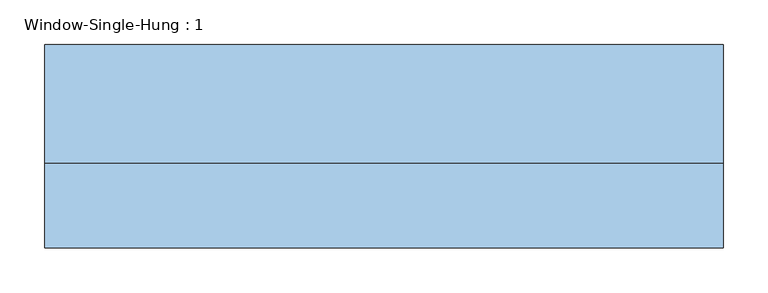
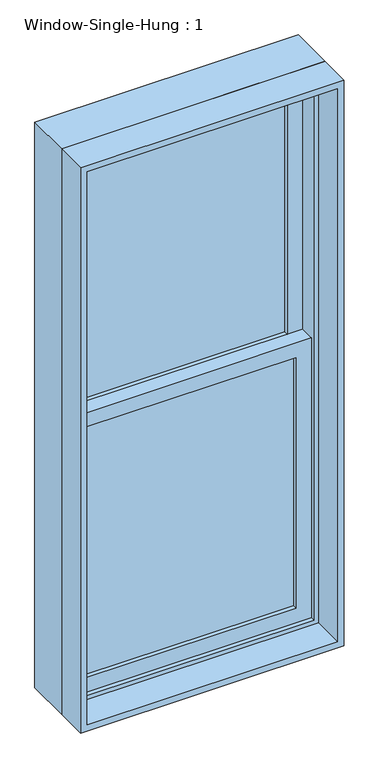
"""IFC4 building model written with IfcOpenShell, lengths in millimetres: window geometry, Window-Single-Hung : 1."""

from ifc_helpers import new_model, si_unit, frame, origin, place, context, project, spatial, polyline, outline, extrude, source, transform, mapped, element, save


def window_single_hung_1_e4cebbcb(model_context):
    return source(origin(), model_context, "Body", "SweptSolid", [
        extrude(outline(polyline([(304.8, 34.925), (304.8, 28.575), (-304.8, 28.575), (-304.8, 34.925), (304.8, 34.925)])), frame((0.0, 0.0, 990.6), z_axis=(0.0, 0.0, 1.0), x_axis=(1.0, 0.0, 0.0)), (0.0, 0.0, 1.0), 765.175),
        extrude(outline(polyline([(-304.8, 22.225), (304.8, 22.225), (304.8, 15.875), (-304.8, 15.875), (-304.8, 22.225)])), frame((0.0, 0.0, 990.6), z_axis=(0.0, 0.0, 1.0), x_axis=(1.0, 0.0, 0.0)), (0.0, 0.0, 1.0), 765.175),
        extrude(outline(polyline([(304.8, 79.375), (304.8, 73.025), (-304.8, 73.025), (-304.8, 79.375), (304.8, 79.375)])), frame((0.0, 0.0, 1800.225), z_axis=(0.0, 0.0, 1.0), x_axis=(1.0, 0.0, 0.0)), (0.0, 0.0, 1.0), 765.175),
        extrude(outline(polyline([(-304.8, 66.675), (304.8, 66.675), (304.8, 60.325), (-304.8, 60.325), (-304.8, 66.675)])), frame((0.0, 0.0, 1800.225), z_axis=(0.0, 0.0, 1.0), x_axis=(1.0, 0.0, 0.0)), (0.0, 0.0, 1.0), 765.175),
        extrude(outline(polyline([(1800.225, -349.25), (946.15, -349.25), (946.15, 349.25), (1800.225, 349.25), (1800.225, -349.25)]), holes=[polyline([(1755.775, 304.8), (990.6, 304.8), (990.6, -304.8), (1755.775, -304.8), (1755.775, 304.8)])]), frame((0.0, 3.175, 0.0), z_axis=(0.0, 1.0, 0.0), x_axis=(0.0, 0.0, 1.0)), (0.0, 0.0, 1.0), 44.45),
        extrude(outline(polyline([(2609.85, -349.25), (1755.775, -349.25), (1755.775, 349.25), (2609.85, 349.25), (2609.85, -349.25)]), holes=[polyline([(2565.4, 304.8), (1800.225, 304.8), (1800.225, -304.8), (2565.4, -304.8), (2565.4, 304.8)])]), frame((0.0, 47.625, 0.0), z_axis=(0.0, 1.0, 0.0), x_axis=(0.0, 0.0, 1.0)), (0.0, 0.0, 1.0), 44.45),
        extrude(outline(polyline([(2641.6, -381.0), (914.4, -381.0), (914.4, 381.0), (2641.6, 381.0), (2641.6, -381.0)]), holes=[polyline([(2609.85, 349.25), (946.15, 349.25), (946.15, -349.25), (2609.85, -349.25), (2609.85, 349.25)])]), frame((0.0, -9.525, 0.0), z_axis=(0.0, 1.0, 0.0), x_axis=(0.0, 0.0, 1.0)), (0.0, 0.0, 1.0), 133.35),
        extrude(outline(polyline([(2641.6, 381.0), (2641.6, -381.0), (914.4, -381.0), (914.4, 381.0), (2641.6, 381.0)]), holes=[polyline([(2622.55, 361.95), (933.45, 361.95), (933.45, -361.95), (2622.55, -361.95), (2622.55, 361.95)])]), frame((0.0, -104.775, 0.0), z_axis=(0.0, 1.0, 0.0), x_axis=(0.0, 0.0, 1.0)), (0.0, 0.0, 1.0), 95.25),
    ])


if __name__ == "__main__":
    model = new_model("IFC4")
    model_context = context("Model", 3, world=origin())
    ifc_project = project(units=[si_unit("LENGTHUNIT", "METRE", prefix="MILLI")], contexts=[model_context])
    site = spatial("IfcSite", under=ifc_project)
    building = spatial("IfcBuilding", under=site)
    placement = place(None, origin())
    window_single_hung_1_shape = window_single_hung_1_e4cebbcb(model_context)
    element("IfcWindow", 1, ObjectType="Window-Single-Hung : 1", at=placement, inside=building, context=model_context, shape_type="MappedRepresentation", body=[
        mapped(window_single_hung_1_shape, transform((0.0, 0.0, 0.0), x_axis=(1.0, 0.0, 0.0), y_axis=(0.0, 1.0, 0.0), z_axis=(0.0, 0.0, 1.0))),
    ])
    save(model, "model.ifc")

# Revit data of these elements
# Type "Window-Single-Hung : 1"
#   Type Mark = "12"
#   Fire Rating = "0.5h"
#   Construction Type Id = "DG-DR"
#   Assembly Code = "B2020100"
#   Analytic Construction = "Double glazing - domestic"
#   Wall Thickness [instance default] = 0' - 6"
#   Window Inset [instance default] = 0' - 0"
#   Visual Light Transmittance = 0.81
#   Thermal Resistance (R) = 0.319569 (m²·K)/W
#   Solar Heat Gain Coefficient = 0.76
#   Muntin Width = 2' - 0"
#   Muntin Height = 2' - 6 1/8"
#   Interior Wall Closure [instance default] = 0' - 1 1/2"
#   Rough Width = 2' - 6 1/2"
#   Rough Height = 5' - 8 1/2"
#   Frame Extension [instance default] = 0' - 1 1/4"
#   Exterior Wall Closure [instance default] = 0' - 0 1/2"
#   Extension Jamb [instance default] = 0' - 1 1/2"
#   Heat Transfer Coefficient (U) = 3.12929 W/(m²·K)
#   Height = 5' - 8"
#   Width = 2' - 6"
#   Top Muntin Visibility = yes
#   Indicator Visibility = no
#   Extension Jamb Visibility [instance default] = yes
#   Interior Trim Visibility [instance default] = yes
#   Exterior Trim Visibility [instance default] = yes
#   Bottom Muntin Visibility = no
#   Muntin Pattern = Muntin Pattern_2x2 : Muntin Pattern_2x2
#   Interior Trim Material = 1X WOOD COMPOSITE TRIM
#   Interior Trim = Trim-Window-Interior-Flat : Picture Frame
#   Exterior Trim Material = 1X WOOD COMPOSITE TRIM
#   Exterior Trim = Trim-Window-Exterior-Flat : with Sill
#   Glass Panel Material = NEW DOUBLE HUNG WINDOWS (TYP.)
#   Exterior Frame Material = 1X WOOD COMPOSITE TRIM
#   Interior Frame Material = 1X WOOD COMPOSITE TRIM
#   Wall Closure = (empty or 0)
# Element 1 (IfcWindow, "Window-Single-Hung : 1")
#   Wall Thickness = 0' - 8 1/4"
#   Extension Jamb = 0' - 3 3/4"
#   Materials on its faces: "1X WOOD COMPOSITE TRIM", "NEW DOUBLE HUNG WINDOWS (TYP.)"
# Materials
#   "1X WOOD COMPOSITE TRIM": class "Generic", colour RGB 88 61 61, transparency 0, Cost = 0
#   "NEW DOUBLE HUNG WINDOWS (TYP.)": class "Glass", colour RGB 218 227 224, transparency 0.85, Description = "Soda Lime Glass", Cost = 0
